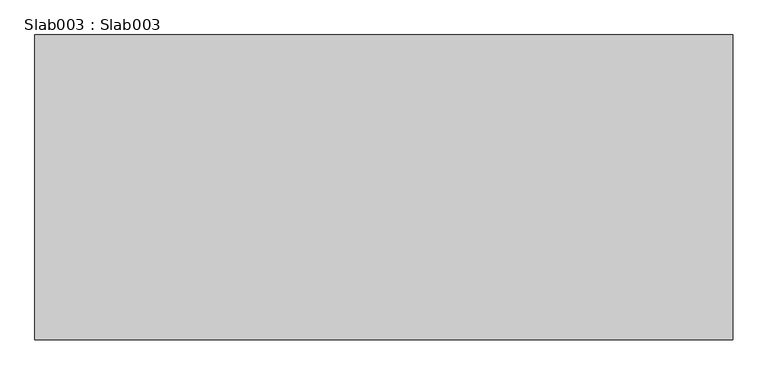
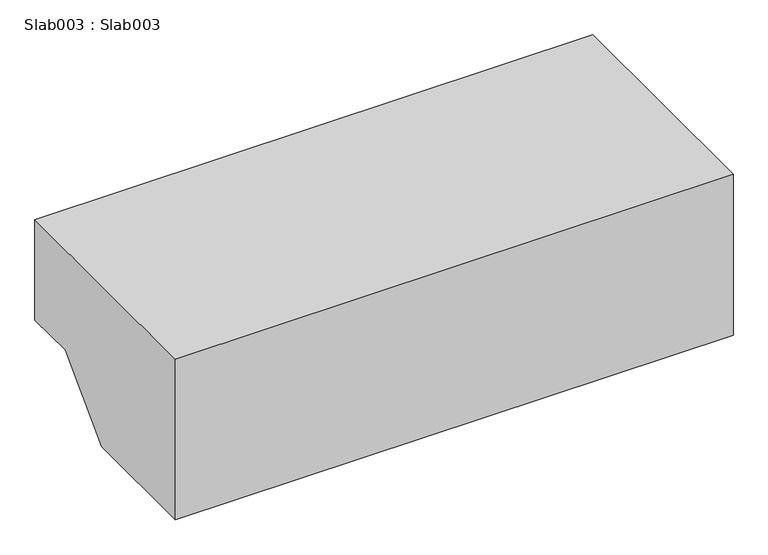
"""IFC4 building model written with IfcOpenShell, lengths in millimetres: proxy geometry, Slab003 : Slab003."""

from ifc_helpers import new_model, si_unit, frame, origin, place, context, project, spatial, polyline, outline, extrude, source, transform, mapped, element, save


def slab003_slab003_1d21d651(model_context):
    return source(origin(), model_context, "Body", "SweptSolid", [
        extrude(outline(polyline([(-4681.9917972, 36531.296), (-3809.2480951, 36531.296), (-3809.2480951, 36150.296), (-3996.1917972, 36150.296), (-4224.7917972, 35921.696), (-4681.9917972, 35921.696), (-4681.9917972, 36531.296)])), frame((12383.0178845, 0.0, 0.0), z_axis=(1.0, 0.0, 0.0), x_axis=(0.0, 1.0, 0.0)), (0.0, 0.0, 1.0), 2000.0),
    ])


if __name__ == "__main__":
    model = new_model("IFC4")
    model_context = context("Model", 3, world=origin())
    ifc_project = project(units=[si_unit("LENGTHUNIT", "METRE", prefix="MILLI")], contexts=[model_context])
    site = spatial("IfcSite", under=ifc_project)
    building = spatial("IfcBuilding", under=site)
    placement = place(None, origin())
    slab003_slab003_shape = slab003_slab003_1d21d651(model_context)
    element("IfcBuildingElementProxy", 1, Name="Slab003 : Slab003", ObjectType="Slab003 : Slab003", at=placement, inside=building, context=model_context, shape_type="MappedRepresentation", body=[
        mapped(slab003_slab003_shape, transform((0.0, 0.0, 0.0), x_axis=(1.0, 0.0, 0.0), y_axis=(0.0, 1.0, 0.0), z_axis=(0.0, 0.0, 1.0))),
    ])
    save(model, "model.ifc")

# Revit data of these elements
# Type "Slab003 : Slab003"
#   NameOverride = "Slab003"
# Element 1 (IfcBuildingElementProxy, "Slab003 : Slab003")
#   Materials on its faces: "CONCRETE SLAB W/ GRADE BEAM (SEE STRUCT DWGS)"
# Materials
#   "CONCRETE SLAB W/ GRADE BEAM (SEE STRUCT DWGS)": class "Unassigned", colour RGB 128 128 128, transparency 0, Cost = 0
